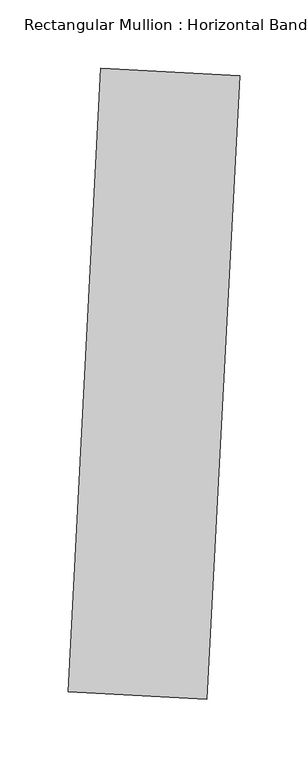
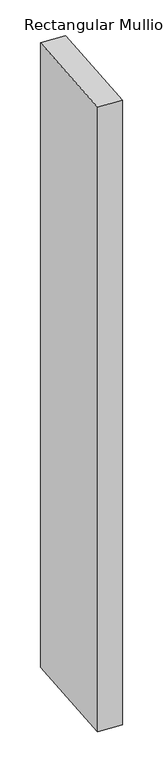
"""IFC4 building model written with IfcOpenShell, lengths in millimetres: member geometry, Rectangular Mullion : Horizontal Band."""

import ifcopenshell
import ifcopenshell.guid

model = None  # the IFC model being written
_history = None  # IfcOwnerHistory: only IFC2X3 demands one
_inside = {}  # id of a spatial element -> (the spatial element, [elements in it])
_under = {}  # id of a project, library or spatial element -> (it, [spatial elements below it])
_declared = {}  # id of a project -> (the project, [libraries it declares])
_typed = {}  # id of a type object -> (the type object, [elements of that type])
_made_of = {}  # id of a material, layer set ... -> (it, [elements and type objects made of it])


def new_model(schema):
    """Start an empty IFC model of exactly this schema.

    Asked for "IFC4X3", IfcOpenShell would pick the latest addendum, in which some entities
    have other attributes; the version numbers below select the first issue.
    IFC2X3 requires an IfcOwnerHistory on every rooted entity: one is made here for all.
    """
    global model, _history
    if schema == "IFC4X3":
        model = ifcopenshell.file(schema_version=(4, 3, 0, 0))
    else:
        model = ifcopenshell.file(schema=schema)
    _inside.clear()
    _under.clear()
    _declared.clear()
    _typed.clear()
    _made_of.clear()
    _history = None
    if model.schema == "IFC2X3":
        org = make("IfcOrganization", Name="unknown")
        user = make(
            "IfcPersonAndOrganization",
            ThePerson=make("IfcPerson", FamilyName="unknown"),
            TheOrganization=org,
        )
        app = make(
            "IfcApplication",
            ApplicationDeveloper=org,
            Version="unknown",
            ApplicationFullName="unknown",
            ApplicationIdentifier="unknown",
        )
        _history = make(
            "IfcOwnerHistory",
            OwningUser=user,
            OwningApplication=app,
            ChangeAction="ADDED",
            CreationDate=0,
        )
    return model


def make(cls, **values):
    """One entity of the class cls with the attributes given. An attribute that is None is left unset."""
    return model.create_entity(
        cls, **{name: value for name, value in values.items() if value is not None}
    )


def rooted(cls, **values):
    """An entity with a GlobalId (a new one), such as an element, a storey or a relation."""
    return make(cls, GlobalId=ifcopenshell.guid.new(), OwnerHistory=_history, **values)


def si_unit(unit_type, name, prefix=None):
    """IfcSIUnit, for example si_unit("LENGTHUNIT", "METRE", prefix="MILLI")."""
    return make("IfcSIUnit", UnitType=unit_type, Prefix=prefix, Name=name)


def assignment(units):
    """IfcUnitAssignment: the units of a project."""
    return None if units is None else make("IfcUnitAssignment", Units=units)


def point(xyz):
    """IfcCartesianPoint."""
    return None if xyz is None else make("IfcCartesianPoint", Coordinates=xyz)


def direction(xyz):
    """IfcDirection."""
    return None if xyz is None else make("IfcDirection", DirectionRatios=xyz)


def frame(location, z_axis=None, x_axis=None):
    """IfcAxis2Placement3D, a coordinate frame: its origin and axes. An axis left out is left unset."""
    return make(
        "IfcAxis2Placement3D",
        Location=point(location),
        Axis=direction(z_axis),
        RefDirection=direction(x_axis),
    )


def origin():
    """The frame at (0, 0, 0) with its axes left unset."""
    return frame((0.0, 0.0, 0.0))


def place(relative_to, where):
    """IfcLocalPlacement: puts the frame where relative to a parent placement (None: the world)."""
    return make(
        "IfcLocalPlacement", PlacementRelTo=relative_to, RelativePlacement=where
    )


def context(
    kind, dimensions, precision=None, world=None, true_north=None, identifier=None
):
    """IfcGeometricRepresentationContext, for example the 3D "Model" context."""
    return make(
        "IfcGeometricRepresentationContext",
        ContextIdentifier=identifier,
        ContextType=kind,
        CoordinateSpaceDimension=dimensions,
        Precision=precision,
        WorldCoordinateSystem=world,
        TrueNorth=true_north,
    )


def project(units=None, contexts=None):
    """IfcProject with its units and contexts."""
    return rooted(
        "IfcProject",
        Name="project",
        RepresentationContexts=contexts,
        UnitsInContext=assignment(units),
    )


def spatial(cls, under=None, at=None, **own):
    """A site, building, storey or space (cls), placed at a placement, below another one or the project."""
    s = rooted(cls, ObjectPlacement=at, **own)
    if under is not None:
        _under.setdefault(under.id(), (under, []))[1].append(s)
    return s


def polyline(points):
    """IfcPolyline through the points."""
    return make("IfcPolyline", Points=[point(p) for p in points])


def outline(outer, holes=None, kind="AREA"):
    """IfcArbitraryClosedProfileDef: a profile drawn as a closed curve; with holes, ...WithVoids."""
    if holes is None:
        return make("IfcArbitraryClosedProfileDef", ProfileType=kind, OuterCurve=outer)
    return make(
        "IfcArbitraryProfileDefWithVoids",
        ProfileType=kind,
        OuterCurve=outer,
        InnerCurves=holes,
    )


def extrude(swept, where, along, depth):
    """IfcExtrudedAreaSolid: the profile swept, set in the frame where, extruded along a direction by depth."""
    return make(
        "IfcExtrudedAreaSolid",
        SweptArea=swept,
        Position=where,
        ExtrudedDirection=direction(along),
        Depth=depth,
    )


def shape(context_of_items, identifier, shape_type, items):
    """IfcShapeRepresentation: the items that make up one representation, for example the "Body"."""
    return make(
        "IfcShapeRepresentation",
        ContextOfItems=context_of_items,
        RepresentationIdentifier=identifier,
        RepresentationType=shape_type,
        Items=items,
    )


def source(mapping_origin, context_of_items, identifier, shape_type, items):
    """IfcRepresentationMap: a shape defined once, which mapped items show again and again."""
    return make(
        "IfcRepresentationMap",
        MappingOrigin=mapping_origin,
        MappedRepresentation=shape(context_of_items, identifier, shape_type, items),
    )


def transform(
    local_origin,
    x_axis=None,
    y_axis=None,
    z_axis=None,
    scale=None,
    scale2=None,
    scale3=None,
    uniform=True,
):
    """IfcCartesianTransformationOperator3D, or its non-uniform kind. x_axis, y_axis, z_axis: its Axis1, 2, 3."""
    if uniform:
        return make(
            "IfcCartesianTransformationOperator3D",
            Axis1=direction(x_axis),
            Axis2=direction(y_axis),
            LocalOrigin=point(local_origin),
            Scale=scale,
            Axis3=direction(z_axis),
        )
    return make(
        "IfcCartesianTransformationOperator3DnonUniform",
        Axis1=direction(x_axis),
        Axis2=direction(y_axis),
        LocalOrigin=point(local_origin),
        Scale=scale,
        Axis3=direction(z_axis),
        Scale2=scale2,
        Scale3=scale3,
    )


def mapped(mapping_source, mapping_target):
    """IfcMappedItem: shows the shape of a source again, moved by a transform."""
    return make(
        "IfcMappedItem", MappingSource=mapping_source, MappingTarget=mapping_target
    )


def made_of(thing, what):
    """Note that an element or type object is made of a material, layer set ...; save() writes the relation."""
    if what is not None:
        _made_of.setdefault(what.id(), (what, []))[1].append(thing)
    return thing


def element(
    cls,
    number,
    at=None,
    inside=None,
    cuts=None,
    type_object=None,
    material=None,
    context=None,
    identifier="Body",
    shape_type=None,
    held_by="IfcProductDefinitionShape",
    body=None,
    shapes=None,
    **own,
):
    """One element of the class cls, such as IfcWall. Its Tag is "e" and its number.

    at: its placement. inside: the storey or other place that contains it. cuts: it is an
    opening in that element (IfcRelVoidsElement). A single representation is given by context,
    identifier, shape_type and body (its items); several are given by shapes. held_by: the class
    of the entity that holds the representations. save() writes the other relations.
    """
    e = rooted(cls, Tag="e%d" % number, ObjectPlacement=at, **own)
    if body is not None:
        shapes = [shape(context, identifier, shape_type, body)]
    if shapes is not None:
        e.Representation = make(held_by, Representations=shapes)
    if inside is not None:
        _inside.setdefault(inside.id(), (inside, []))[1].append(e)
    if cuts is not None:
        rooted(
            "IfcRelVoidsElement", RelatingBuildingElement=cuts, RelatedOpeningElement=e
        )
    if type_object is not None:
        _typed.setdefault(type_object.id(), (type_object, []))[1].append(e)
    return made_of(e, material)


def aggregate(whole, parts):
    """IfcRelAggregates: a whole, such as a stair, and the parts it consists of."""
    return rooted("IfcRelAggregates", RelatingObject=whole, RelatedObjects=parts)


def save(model, path):
    """Write the relations noted so far, then the file.

    IfcRelAggregates (storeys below a building ...), IfcRelContainedInSpatialStructure (elements
    in a storey), IfcRelDefinesByType, IfcRelAssociatesMaterial and IfcRelDeclares: one each for
    every whole, place, type object, material and project.
    """
    for whole, parts in _under.values():
        aggregate(whole, parts)
    for where, things in _inside.values():
        rooted(
            "IfcRelContainedInSpatialStructure",
            RelatedElements=things,
            RelatingStructure=where,
        )
    for kind, things in _typed.values():
        rooted("IfcRelDefinesByType", RelatedObjects=things, RelatingType=kind)
    for what, things in _made_of.values():
        rooted("IfcRelAssociatesMaterial", RelatedObjects=things, RelatingMaterial=what)
    for by, libraries in _declared.values():
        rooted("IfcRelDeclares", RelatingContext=by, RelatedDefinitions=libraries)
    model.write(path)


def rectangular_mullion_horizontal_band_1f6ee450(model_context):
    return source(origin(), model_context, "Body", "SweptSolid", [
        extrude(outline(polyline([(62.69438, 301.8280451), (38.7663808, -154.7453782), (-62.69438, -149.4280451), (-38.7663808, 307.1453782), (62.69438, 301.8280451)])), frame((0.0, 0.0, -2765.4069854), z_axis=(0.0, 0.0, 1.0), x_axis=(1.0, 0.0, 0.0)), (0.0, 0.0, 1.0), 2765.4069854),
    ])


if __name__ == "__main__":
    model = new_model("IFC4")
    model_context = context("Model", 3, world=origin())
    ifc_project = project(units=[si_unit("LENGTHUNIT", "METRE", prefix="MILLI")], contexts=[model_context])
    site = spatial("IfcSite", under=ifc_project)
    building = spatial("IfcBuilding", under=site)
    placement = place(None, origin())
    rectangular_mullion_horizontal_band_shape = rectangular_mullion_horizontal_band_1f6ee450(model_context)
    element("IfcMember", 1, ObjectType="Rectangular Mullion : Horizontal Band", at=placement, inside=building, context=model_context, shape_type="MappedRepresentation", body=[
        mapped(rectangular_mullion_horizontal_band_shape, transform((0.0, 0.0, 0.0), x_axis=(1.0, 0.0, 0.0), y_axis=(0.0, 1.0, 0.0), z_axis=(0.0, 0.0, 1.0))),
    ])
    save(model, "model.ifc")

# Revit data of these elements
# Project information
#   Organization Name = "G3B Press"
#   Organization Description = "Paul F. Aubin Cosulting Services, Inc."
#   Building Name = "Revit Essentials for Architecture"
#   Author = "Paul F. Aubin"
#   Author Website = "https://www.paulaubin.com"
#   Copyright = "Copyright © 2020 Paul F Aubin, all rights reserved"
#   Design Option = "Main Model"
#   Project Issue Date = "8/1/2020"
#   Project Status = "Design Development"
#   Client Name = "Ceiling Plans and Interior Elevations"
#   Project Address = "123 State ST\nSuite 301\nChicago, IL 60606"
#   Project Name = "14 Commercial"
#   Project Number = "2020.04A"
# Type "Rectangular Mullion : Horizontal Band"
#   built-in parameter 1007351 = 0.25 (stored number, unit not read)
#   built-in parameter 1007304 = 1.5 (stored number, unit not read)
#   built-in parameter 1007301 = 0.166667 (stored number, unit not read)
#   built-in parameter 1007300 = 0.166667 (stored number, unit not read)
# Element 1 (IfcMember, "Rectangular Mullion : Horizontal Band")
#   Materials on its faces: "Aluminum"
# Materials
#   "Aluminum": class "Metal", colour RGB 247 247 247, transparency 0, Description = "Aluminum 6061", Cost = 0
